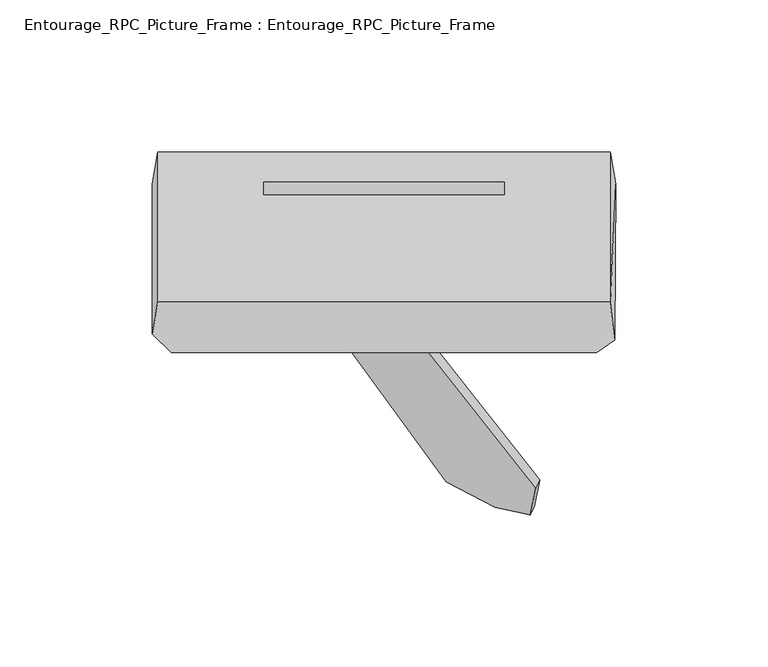
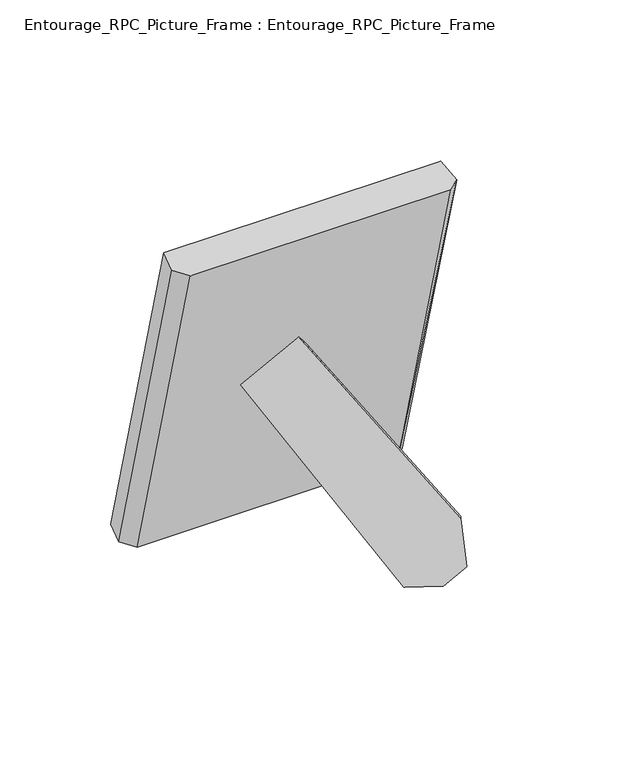
"""IFC4 building model written with IfcOpenShell, lengths in millimetres: proxy geometry, Entourage_RPC_Picture_Frame : Entourage_RPC_Picture_Frame."""

import ifcopenshell
import ifcopenshell.guid

model = None  # the IFC model being written
_history = None  # IfcOwnerHistory: only IFC2X3 demands one
_inside = {}  # id of a spatial element -> (the spatial element, [elements in it])
_under = {}  # id of a project, library or spatial element -> (it, [spatial elements below it])
_declared = {}  # id of a project -> (the project, [libraries it declares])
_typed = {}  # id of a type object -> (the type object, [elements of that type])
_made_of = {}  # id of a material, layer set ... -> (it, [elements and type objects made of it])


def new_model(schema):
    """Start an empty IFC model of exactly this schema.

    Asked for "IFC4X3", IfcOpenShell would pick the latest addendum, in which some entities
    have other attributes; the version numbers below select the first issue.
    IFC2X3 requires an IfcOwnerHistory on every rooted entity: one is made here for all.
    """
    global model, _history
    if schema == "IFC4X3":
        model = ifcopenshell.file(schema_version=(4, 3, 0, 0))
    else:
        model = ifcopenshell.file(schema=schema)
    _inside.clear()
    _under.clear()
    _declared.clear()
    _typed.clear()
    _made_of.clear()
    _history = None
    if model.schema == "IFC2X3":
        org = make("IfcOrganization", Name="unknown")
        user = make(
            "IfcPersonAndOrganization",
            ThePerson=make("IfcPerson", FamilyName="unknown"),
            TheOrganization=org,
        )
        app = make(
            "IfcApplication",
            ApplicationDeveloper=org,
            Version="unknown",
            ApplicationFullName="unknown",
            ApplicationIdentifier="unknown",
        )
        _history = make(
            "IfcOwnerHistory",
            OwningUser=user,
            OwningApplication=app,
            ChangeAction="ADDED",
            CreationDate=0,
        )
    return model


def make(cls, **values):
    """One entity of the class cls with the attributes given. An attribute that is None is left unset."""
    return model.create_entity(
        cls, **{name: value for name, value in values.items() if value is not None}
    )


def rooted(cls, **values):
    """An entity with a GlobalId (a new one), such as an element, a storey or a relation."""
    return make(cls, GlobalId=ifcopenshell.guid.new(), OwnerHistory=_history, **values)


def si_unit(unit_type, name, prefix=None):
    """IfcSIUnit, for example si_unit("LENGTHUNIT", "METRE", prefix="MILLI")."""
    return make("IfcSIUnit", UnitType=unit_type, Prefix=prefix, Name=name)


def assignment(units):
    """IfcUnitAssignment: the units of a project."""
    return None if units is None else make("IfcUnitAssignment", Units=units)


def point(xyz):
    """IfcCartesianPoint."""
    return None if xyz is None else make("IfcCartesianPoint", Coordinates=xyz)


def direction(xyz):
    """IfcDirection."""
    return None if xyz is None else make("IfcDirection", DirectionRatios=xyz)


def frame(location, z_axis=None, x_axis=None):
    """IfcAxis2Placement3D, a coordinate frame: its origin and axes. An axis left out is left unset."""
    return make(
        "IfcAxis2Placement3D",
        Location=point(location),
        Axis=direction(z_axis),
        RefDirection=direction(x_axis),
    )


def origin():
    """The frame at (0, 0, 0) with its axes left unset."""
    return frame((0.0, 0.0, 0.0))


def place(relative_to, where):
    """IfcLocalPlacement: puts the frame where relative to a parent placement (None: the world)."""
    return make(
        "IfcLocalPlacement", PlacementRelTo=relative_to, RelativePlacement=where
    )


def context(
    kind, dimensions, precision=None, world=None, true_north=None, identifier=None
):
    """IfcGeometricRepresentationContext, for example the 3D "Model" context."""
    return make(
        "IfcGeometricRepresentationContext",
        ContextIdentifier=identifier,
        ContextType=kind,
        CoordinateSpaceDimension=dimensions,
        Precision=precision,
        WorldCoordinateSystem=world,
        TrueNorth=true_north,
    )


def project(units=None, contexts=None):
    """IfcProject with its units and contexts."""
    return rooted(
        "IfcProject",
        Name="project",
        RepresentationContexts=contexts,
        UnitsInContext=assignment(units),
    )


def spatial(cls, under=None, at=None, **own):
    """A site, building, storey or space (cls), placed at a placement, below another one or the project."""
    s = rooted(cls, ObjectPlacement=at, **own)
    if under is not None:
        _under.setdefault(under.id(), (under, []))[1].append(s)
    return s


def point_list(points):
    """IfcCartesianPointList2D or 3D."""
    cls = (
        "IfcCartesianPointList2D" if len(points[0]) == 2 else "IfcCartesianPointList3D"
    )
    return make(cls, CoordList=points)


def triangles(points, corners, closed=None, point_numbers=None):
    """IfcTriangulatedFaceSet: each triangle names its three corners, points numbered from 1."""
    return make(
        "IfcTriangulatedFaceSet",
        Coordinates=point_list(points),
        Closed=closed,
        CoordIndex=corners,
        PnIndex=point_numbers,
    )


def shape(context_of_items, identifier, shape_type, items):
    """IfcShapeRepresentation: the items that make up one representation, for example the "Body"."""
    return make(
        "IfcShapeRepresentation",
        ContextOfItems=context_of_items,
        RepresentationIdentifier=identifier,
        RepresentationType=shape_type,
        Items=items,
    )


def source(mapping_origin, context_of_items, identifier, shape_type, items):
    """IfcRepresentationMap: a shape defined once, which mapped items show again and again."""
    return make(
        "IfcRepresentationMap",
        MappingOrigin=mapping_origin,
        MappedRepresentation=shape(context_of_items, identifier, shape_type, items),
    )


def transform(
    local_origin,
    x_axis=None,
    y_axis=None,
    z_axis=None,
    scale=None,
    scale2=None,
    scale3=None,
    uniform=True,
):
    """IfcCartesianTransformationOperator3D, or its non-uniform kind. x_axis, y_axis, z_axis: its Axis1, 2, 3."""
    if uniform:
        return make(
            "IfcCartesianTransformationOperator3D",
            Axis1=direction(x_axis),
            Axis2=direction(y_axis),
            LocalOrigin=point(local_origin),
            Scale=scale,
            Axis3=direction(z_axis),
        )
    return make(
        "IfcCartesianTransformationOperator3DnonUniform",
        Axis1=direction(x_axis),
        Axis2=direction(y_axis),
        LocalOrigin=point(local_origin),
        Scale=scale,
        Axis3=direction(z_axis),
        Scale2=scale2,
        Scale3=scale3,
    )


def mapped(mapping_source, mapping_target):
    """IfcMappedItem: shows the shape of a source again, moved by a transform."""
    return make(
        "IfcMappedItem", MappingSource=mapping_source, MappingTarget=mapping_target
    )


def made_of(thing, what):
    """Note that an element or type object is made of a material, layer set ...; save() writes the relation."""
    if what is not None:
        _made_of.setdefault(what.id(), (what, []))[1].append(thing)
    return thing


def element(
    cls,
    number,
    at=None,
    inside=None,
    cuts=None,
    type_object=None,
    material=None,
    context=None,
    identifier="Body",
    shape_type=None,
    held_by="IfcProductDefinitionShape",
    body=None,
    shapes=None,
    **own,
):
    """One element of the class cls, such as IfcWall. Its Tag is "e" and its number.

    at: its placement. inside: the storey or other place that contains it. cuts: it is an
    opening in that element (IfcRelVoidsElement). A single representation is given by context,
    identifier, shape_type and body (its items); several are given by shapes. held_by: the class
    of the entity that holds the representations. save() writes the other relations.
    """
    e = rooted(cls, Tag="e%d" % number, ObjectPlacement=at, **own)
    if body is not None:
        shapes = [shape(context, identifier, shape_type, body)]
    if shapes is not None:
        e.Representation = make(held_by, Representations=shapes)
    if inside is not None:
        _inside.setdefault(inside.id(), (inside, []))[1].append(e)
    if cuts is not None:
        rooted(
            "IfcRelVoidsElement", RelatingBuildingElement=cuts, RelatedOpeningElement=e
        )
    if type_object is not None:
        _typed.setdefault(type_object.id(), (type_object, []))[1].append(e)
    return made_of(e, material)


def aggregate(whole, parts):
    """IfcRelAggregates: a whole, such as a stair, and the parts it consists of."""
    return rooted("IfcRelAggregates", RelatingObject=whole, RelatedObjects=parts)


def save(model, path):
    """Write the relations noted so far, then the file.

    IfcRelAggregates (storeys below a building ...), IfcRelContainedInSpatialStructure (elements
    in a storey), IfcRelDefinesByType, IfcRelAssociatesMaterial and IfcRelDeclares: one each for
    every whole, place, type object, material and project.
    """
    for whole, parts in _under.values():
        aggregate(whole, parts)
    for where, things in _inside.values():
        rooted(
            "IfcRelContainedInSpatialStructure",
            RelatedElements=things,
            RelatingStructure=where,
        )
    for kind, things in _typed.values():
        rooted("IfcRelDefinesByType", RelatedObjects=things, RelatingType=kind)
    for what, things in _made_of.values():
        rooted("IfcRelAssociatesMaterial", RelatedObjects=things, RelatingMaterial=what)
    for by, libraries in _declared.values():
        rooted("IfcRelDeclares", RelatingContext=by, RelatedDefinitions=libraries)
    model.write(path)


def entourage_rpc_picture_frame_entourage_rpc_picture_frame_0c3f382a(model_context):
    return source(origin(), model_context, "Body", "Tessellation", [
        triangles([(-31.2212752, 21.3179439, 97.8039775), (-3.3552966, 15.6563572, 118.0830721), (49.8722556, -51.6400711, 31.432093), (48.0637995, -60.4893174, 9.6569551), (36.5907671, -58.1576284, 1.3080831), (20.4721357, -49.6588966, 1.1709248), (-29.8344526, 23.9264897, 96.6279682), (-1.9710145, 18.262363, 116.9070629), (51.2565371, -49.0391442, 30.2611684), (49.4455375, -57.8858517, 8.4834904), (37.9725073, -55.5541626, 0.1346183), (21.8564171, -47.0554308, -0.00254), (-74.3118158, 9.430898, 188.4655675), (74.3118158, 9.430898, 188.4655675), (75.7926166, -3.1317793, 185.1001116), (69.8490931, -7.2160464, 184.0053746), (-69.8490931, -7.2160464, 184.0053746), (-76.1990144, -1.082026, 185.6487336), (-74.3118158, 58.7342011, 4.4601824), (74.3118158, 58.7469002, 4.4398626), (76.1990144, 48.2212754, 1.6433587), (69.8490931, 42.0897955, 0.0), (-69.8490931, 42.0897955, 0.0), (-76.1990144, 48.2212754, 1.6433587), (-39.6869853, 19.0954732, 152.4335917), (39.6869853, 19.0954732, 152.436117), (39.6869853, 49.0899451, 40.4972374), (-39.6869853, 49.0899451, 40.4972374), (-39.6869853, 14.7064095, 151.2575824), (39.6869853, 14.7064095, 151.2575824), (39.6869853, 44.7008825, 39.3212327), (-39.6869853, 44.7008825, 39.3212327)], [[1, 2, 8], [1, 8, 7], [2, 3, 9], [2, 9, 8], [3, 4, 10], [3, 10, 9], [4, 5, 11], [4, 11, 10], [5, 6, 12], [5, 12, 11], [6, 1, 7], [6, 7, 12], [1, 3, 2], [6, 3, 1], [6, 4, 3], [5, 4, 6], [7, 8, 9], [12, 7, 9], [12, 9, 10], [11, 12, 10], [15, 17, 16], [14, 17, 15], [13, 17, 14], [18, 17, 13], [21, 22, 23], [20, 21, 23], [19, 20, 23], [24, 19, 23], [23, 22, 16], [16, 17, 23], [20, 19, 27], [27, 19, 28], [14, 25, 13], [26, 25, 14], [14, 20, 27], [27, 26, 14], [28, 19, 13], [13, 25, 28], [29, 32, 28], [28, 25, 29], [30, 29, 25], [25, 26, 30], [31, 30, 26], [26, 27, 31], [32, 31, 27], [27, 28, 32], [31, 32, 29], [30, 31, 29], [14, 15, 21], [14, 21, 20], [15, 16, 22], [15, 22, 21], [17, 18, 24], [17, 24, 23], [18, 13, 19], [18, 19, 24]]),
    ])


if __name__ == "__main__":
    model = new_model("IFC4")
    model_context = context("Model", 3, world=origin())
    ifc_project = project(units=[si_unit("LENGTHUNIT", "METRE", prefix="MILLI")], contexts=[model_context])
    site = spatial("IfcSite", under=ifc_project)
    building = spatial("IfcBuilding", under=site)
    placement = place(None, origin())
    entourage_rpc_picture_frame_entourage_rpc_picture_frame_shape = entourage_rpc_picture_frame_entourage_rpc_picture_frame_0c3f382a(model_context)
    element("IfcBuildingElementProxy", 1, Name="Entourage_RPC_Picture_Frame : Entourage_RPC_Picture_Frame", ObjectType="Entourage_RPC_Picture_Frame : Entourage_RPC_Picture_Frame", at=placement, inside=building, context=model_context, shape_type="MappedRepresentation", body=[
        mapped(entourage_rpc_picture_frame_entourage_rpc_picture_frame_shape, transform((0.0, 0.0, 0.0), x_axis=(1.0, 0.0, 0.0), y_axis=(0.0, 1.0, 0.0), z_axis=(0.0, 0.0, 1.0))),
    ])
    save(model, "model.ifc")

# Revit data of these elements
# Type "Entourage_RPC_Picture_Frame : Entourage_RPC_Picture_Frame"
#   built-in parameter 1005198 = "{2, 15},{39, RPC-16-8M5E-0H3T-F0AH-3U0K-JLQ7-G28B-AU},{1, 0},{1, 0},{2, 19},{1, 8},{5, Color},{1, 0},{1, 0},{3, 0.8},{3, 0.8},{3, 0.8},{1, 8},{7, BBoxMin},{1, 0},{1, 0},{1, 0},{1, 0},{1, 0},{1, 8},{7, BBoxMax},{1, 0},{1, 0},{1, 0},{1, 0},{1, 0},{2, 11},{9, RPCTypeId},{1, 0},{1, 0},{39, RPC-16-8M5E-0H3T-F0AH-3U0K-JLQ7-G28B-AU},{1, 6},{14, RPCPlantHeight},{1, 0},{1, 0},{8, 0.624409},{2, 11},{7, keyword},{1, 0},{1, 0},{33, :RPCs:Office Clutter:Geometry:RPC},{2, 11},{8, category},{1, 0},{1, 0},{14, Office Clutter},{2, 11},{12, LocalizedUID},{1, 0},{1, 0},{13, Picture Frame},{2, 14},{6, Height},{1, 0},{1, 0},{8, 0.624409},{1, 2},{16, Cast Reflections},{1, 0},{1, 0},{1, 0},{1, 2},{8, Portrait},{1, 0},{1, 0},{1, 1},{1, 2},{5, Stand},{1, 0},{1, 0},{1, 1},{2, 11},{10, RPCL_Frame},{1, 0},{1, 0},{5, Frame},{1, 4},{14, Frame Material},{1, 0},{1, 0},{1, 0},{2, 11},{12, RPCL_Picture},{1, 0},{1, 0},{7, Picture},{2, 11},{15, Picture Preview},{1, 0},{1, 0},{65, __RPC:/object data/textures/object/Photo/Photo0/textures/Portrait},{2, 11},{17, i_Picture Preview},{1, 0},{1, 0},{0, },{1, 2},{18, Use Custom Picture},{1, 0},{1, 0},{1, 0},{2, 11},{17, Picture File Name},{1, 0},{1, 0},{0, },{21, assetlibrary_base.fbx},{1, 5},"
#   built-in parameter 1005195 = "RPC-16-8M5E-0H3T-F0AH-3U0K-JLQ7-G28B-AU"
#   Height = 0
